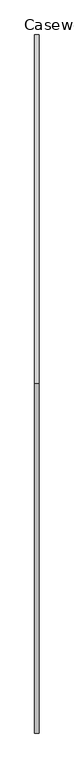
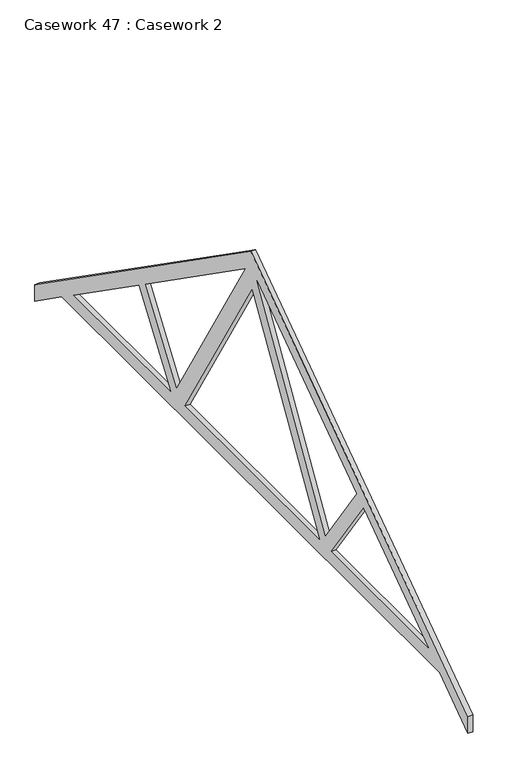
"""IFC4 building model written with IfcOpenShell, lengths in millimetres: furniture geometry, Casework 47 : Casework 2."""

import ifcopenshell
import ifcopenshell.guid

model = None  # the IFC model being written
_history = None  # IfcOwnerHistory: only IFC2X3 demands one
_inside = {}  # id of a spatial element -> (the spatial element, [elements in it])
_under = {}  # id of a project, library or spatial element -> (it, [spatial elements below it])
_declared = {}  # id of a project -> (the project, [libraries it declares])
_typed = {}  # id of a type object -> (the type object, [elements of that type])
_made_of = {}  # id of a material, layer set ... -> (it, [elements and type objects made of it])


def new_model(schema):
    """Start an empty IFC model of exactly this schema.

    Asked for "IFC4X3", IfcOpenShell would pick the latest addendum, in which some entities
    have other attributes; the version numbers below select the first issue.
    IFC2X3 requires an IfcOwnerHistory on every rooted entity: one is made here for all.
    """
    global model, _history
    if schema == "IFC4X3":
        model = ifcopenshell.file(schema_version=(4, 3, 0, 0))
    else:
        model = ifcopenshell.file(schema=schema)
    _inside.clear()
    _under.clear()
    _declared.clear()
    _typed.clear()
    _made_of.clear()
    _history = None
    if model.schema == "IFC2X3":
        org = make("IfcOrganization", Name="unknown")
        user = make(
            "IfcPersonAndOrganization",
            ThePerson=make("IfcPerson", FamilyName="unknown"),
            TheOrganization=org,
        )
        app = make(
            "IfcApplication",
            ApplicationDeveloper=org,
            Version="unknown",
            ApplicationFullName="unknown",
            ApplicationIdentifier="unknown",
        )
        _history = make(
            "IfcOwnerHistory",
            OwningUser=user,
            OwningApplication=app,
            ChangeAction="ADDED",
            CreationDate=0,
        )
    return model


def make(cls, **values):
    """One entity of the class cls with the attributes given. An attribute that is None is left unset."""
    return model.create_entity(
        cls, **{name: value for name, value in values.items() if value is not None}
    )


def rooted(cls, **values):
    """An entity with a GlobalId (a new one), such as an element, a storey or a relation."""
    return make(cls, GlobalId=ifcopenshell.guid.new(), OwnerHistory=_history, **values)


def si_unit(unit_type, name, prefix=None):
    """IfcSIUnit, for example si_unit("LENGTHUNIT", "METRE", prefix="MILLI")."""
    return make("IfcSIUnit", UnitType=unit_type, Prefix=prefix, Name=name)


def assignment(units):
    """IfcUnitAssignment: the units of a project."""
    return None if units is None else make("IfcUnitAssignment", Units=units)


def point(xyz):
    """IfcCartesianPoint."""
    return None if xyz is None else make("IfcCartesianPoint", Coordinates=xyz)


def direction(xyz):
    """IfcDirection."""
    return None if xyz is None else make("IfcDirection", DirectionRatios=xyz)


def frame(location, z_axis=None, x_axis=None):
    """IfcAxis2Placement3D, a coordinate frame: its origin and axes. An axis left out is left unset."""
    return make(
        "IfcAxis2Placement3D",
        Location=point(location),
        Axis=direction(z_axis),
        RefDirection=direction(x_axis),
    )


def origin():
    """The frame at (0, 0, 0) with its axes left unset."""
    return frame((0.0, 0.0, 0.0))


def place(relative_to, where):
    """IfcLocalPlacement: puts the frame where relative to a parent placement (None: the world)."""
    return make(
        "IfcLocalPlacement", PlacementRelTo=relative_to, RelativePlacement=where
    )


def context(
    kind, dimensions, precision=None, world=None, true_north=None, identifier=None
):
    """IfcGeometricRepresentationContext, for example the 3D "Model" context."""
    return make(
        "IfcGeometricRepresentationContext",
        ContextIdentifier=identifier,
        ContextType=kind,
        CoordinateSpaceDimension=dimensions,
        Precision=precision,
        WorldCoordinateSystem=world,
        TrueNorth=true_north,
    )


def project(units=None, contexts=None):
    """IfcProject with its units and contexts."""
    return rooted(
        "IfcProject",
        Name="project",
        RepresentationContexts=contexts,
        UnitsInContext=assignment(units),
    )


def spatial(cls, under=None, at=None, **own):
    """A site, building, storey or space (cls), placed at a placement, below another one or the project."""
    s = rooted(cls, ObjectPlacement=at, **own)
    if under is not None:
        _under.setdefault(under.id(), (under, []))[1].append(s)
    return s


def polyline(points):
    """IfcPolyline through the points."""
    return make("IfcPolyline", Points=[point(p) for p in points])


def outline(outer, holes=None, kind="AREA"):
    """IfcArbitraryClosedProfileDef: a profile drawn as a closed curve; with holes, ...WithVoids."""
    if holes is None:
        return make("IfcArbitraryClosedProfileDef", ProfileType=kind, OuterCurve=outer)
    return make(
        "IfcArbitraryProfileDefWithVoids",
        ProfileType=kind,
        OuterCurve=outer,
        InnerCurves=holes,
    )


def extrude(swept, where, along, depth):
    """IfcExtrudedAreaSolid: the profile swept, set in the frame where, extruded along a direction by depth."""
    return make(
        "IfcExtrudedAreaSolid",
        SweptArea=swept,
        Position=where,
        ExtrudedDirection=direction(along),
        Depth=depth,
    )


def shape(context_of_items, identifier, shape_type, items):
    """IfcShapeRepresentation: the items that make up one representation, for example the "Body"."""
    return make(
        "IfcShapeRepresentation",
        ContextOfItems=context_of_items,
        RepresentationIdentifier=identifier,
        RepresentationType=shape_type,
        Items=items,
    )


def source(mapping_origin, context_of_items, identifier, shape_type, items):
    """IfcRepresentationMap: a shape defined once, which mapped items show again and again."""
    return make(
        "IfcRepresentationMap",
        MappingOrigin=mapping_origin,
        MappedRepresentation=shape(context_of_items, identifier, shape_type, items),
    )


def transform(
    local_origin,
    x_axis=None,
    y_axis=None,
    z_axis=None,
    scale=None,
    scale2=None,
    scale3=None,
    uniform=True,
):
    """IfcCartesianTransformationOperator3D, or its non-uniform kind. x_axis, y_axis, z_axis: its Axis1, 2, 3."""
    if uniform:
        return make(
            "IfcCartesianTransformationOperator3D",
            Axis1=direction(x_axis),
            Axis2=direction(y_axis),
            LocalOrigin=point(local_origin),
            Scale=scale,
            Axis3=direction(z_axis),
        )
    return make(
        "IfcCartesianTransformationOperator3DnonUniform",
        Axis1=direction(x_axis),
        Axis2=direction(y_axis),
        LocalOrigin=point(local_origin),
        Scale=scale,
        Axis3=direction(z_axis),
        Scale2=scale2,
        Scale3=scale3,
    )


def mapped(mapping_source, mapping_target):
    """IfcMappedItem: shows the shape of a source again, moved by a transform."""
    return make(
        "IfcMappedItem", MappingSource=mapping_source, MappingTarget=mapping_target
    )


def made_of(thing, what):
    """Note that an element or type object is made of a material, layer set ...; save() writes the relation."""
    if what is not None:
        _made_of.setdefault(what.id(), (what, []))[1].append(thing)
    return thing


def element(
    cls,
    number,
    at=None,
    inside=None,
    cuts=None,
    type_object=None,
    material=None,
    context=None,
    identifier="Body",
    shape_type=None,
    held_by="IfcProductDefinitionShape",
    body=None,
    shapes=None,
    **own,
):
    """One element of the class cls, such as IfcWall. Its Tag is "e" and its number.

    at: its placement. inside: the storey or other place that contains it. cuts: it is an
    opening in that element (IfcRelVoidsElement). A single representation is given by context,
    identifier, shape_type and body (its items); several are given by shapes. held_by: the class
    of the entity that holds the representations. save() writes the other relations.
    """
    e = rooted(cls, Tag="e%d" % number, ObjectPlacement=at, **own)
    if body is not None:
        shapes = [shape(context, identifier, shape_type, body)]
    if shapes is not None:
        e.Representation = make(held_by, Representations=shapes)
    if inside is not None:
        _inside.setdefault(inside.id(), (inside, []))[1].append(e)
    if cuts is not None:
        rooted(
            "IfcRelVoidsElement", RelatingBuildingElement=cuts, RelatedOpeningElement=e
        )
    if type_object is not None:
        _typed.setdefault(type_object.id(), (type_object, []))[1].append(e)
    return made_of(e, material)


def aggregate(whole, parts):
    """IfcRelAggregates: a whole, such as a stair, and the parts it consists of."""
    return rooted("IfcRelAggregates", RelatingObject=whole, RelatedObjects=parts)


def save(model, path):
    """Write the relations noted so far, then the file.

    IfcRelAggregates (storeys below a building ...), IfcRelContainedInSpatialStructure (elements
    in a storey), IfcRelDefinesByType, IfcRelAssociatesMaterial and IfcRelDeclares: one each for
    every whole, place, type object, material and project.
    """
    for whole, parts in _under.values():
        aggregate(whole, parts)
    for where, things in _inside.values():
        rooted(
            "IfcRelContainedInSpatialStructure",
            RelatedElements=things,
            RelatingStructure=where,
        )
    for kind, things in _typed.values():
        rooted("IfcRelDefinesByType", RelatedObjects=things, RelatingType=kind)
    for what, things in _made_of.values():
        rooted("IfcRelAssociatesMaterial", RelatedObjects=things, RelatingMaterial=what)
    for by, libraries in _declared.values():
        rooted("IfcRelDeclares", RelatingContext=by, RelatedDefinitions=libraries)
    model.write(path)


def casework_47_casework_2_612639c6(model_context):
    return source(origin(), model_context, "Body", "SweptSolid", [
        extrude(outline(polyline([(6583.1149316, 5265.0), (-277.3850684, 5265.0), (-786.6126654, 4908.4349979), (-786.6126654, 5091.5511862), (3152.8649316, 7850.0030963), (7073.1149316, 5105.0144946), (7073.1149316, 4921.8983063), (6583.1149316, 5265.0)]), holes=[polyline([(4612.3149663, 5415.0), (6368.8927306, 5415.0), (5190.2113591, 6240.3215815), (4612.3149663, 5415.0)]), polyline([(4346.6651995, 5415.0), (3129.0956471, 7441.3760243), (1911.5260948, 5415.0), (4346.6651995, 5415.0)]), polyline([(4504.5438357, 5522.6038939), (5067.3385525, 6326.3580469), (3262.0771677, 7590.415677), (4504.5438357, 5522.6038939)]), polyline([(1693.4148969, 5415.0), (1115.5185041, 6240.3215815), (-63.1628674, 5415.0), (1693.4148969, 5415.0)]), polyline([(1801.1860276, 5522.6038939), (3043.6526956, 7590.415677), (1238.3913108, 6326.3580469), (1801.1860276, 5522.6038939)])]), frame((-10901.5247381, 0.0, 0.0), z_axis=(1.0, 0.0, 0.0), x_axis=(0.0, 1.0, 0.0)), (0.0, 0.0, 1.0), 49.6351915),
    ])


if __name__ == "__main__":
    model = new_model("IFC4")
    model_context = context("Model", 3, world=origin())
    ifc_project = project(units=[si_unit("LENGTHUNIT", "METRE", prefix="MILLI")], contexts=[model_context])
    site = spatial("IfcSite", under=ifc_project)
    building = spatial("IfcBuilding", under=site)
    placement = place(None, origin())
    casework_47_casework_2_shape = casework_47_casework_2_612639c6(model_context)
    element("IfcFurniture", 1, ObjectType="Casework 47 : Casework 2", at=placement, inside=building, context=model_context, shape_type="MappedRepresentation", body=[
        mapped(casework_47_casework_2_shape, transform((0.0, 0.0, 0.0), x_axis=(1.0, 0.0, 0.0), y_axis=(0.0, 1.0, 0.0), z_axis=(0.0, 0.0, 1.0))),
    ])
    save(model, "model.ifc")

# Revit data of these elements
# Element 1 (IfcFurniture, "Casework 47 : Casework 2")
#   Materials on its faces: "Softwood, Lumber"
# Materials
#   "Softwood, Lumber": class "Wood", colour RGB 205 156 65, transparency 0, Description = "Pinus Echinata", Cost = 0
